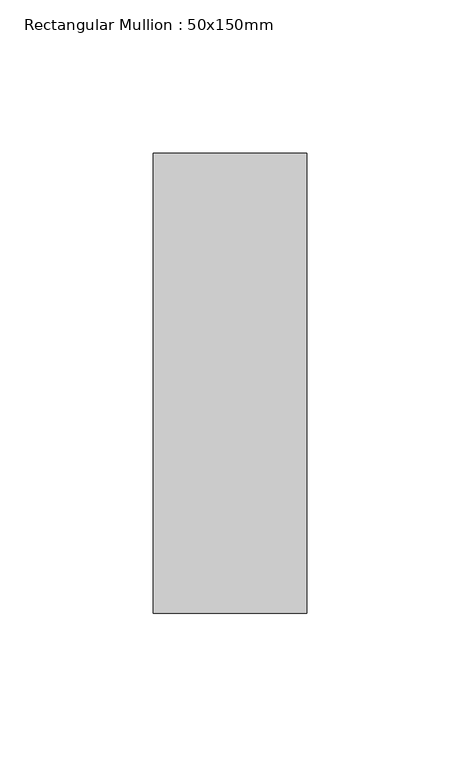
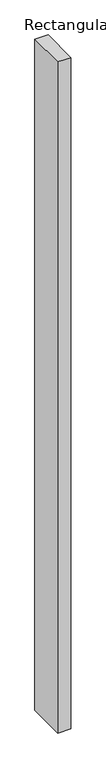
"""IFC4 building model written with IfcOpenShell, lengths in millimetres: member geometry, Rectangular Mullion : 50x150mm."""

import ifcopenshell
import ifcopenshell.guid

model = None  # the IFC model being written
_history = None  # IfcOwnerHistory: only IFC2X3 demands one
_inside = {}  # id of a spatial element -> (the spatial element, [elements in it])
_under = {}  # id of a project, library or spatial element -> (it, [spatial elements below it])
_declared = {}  # id of a project -> (the project, [libraries it declares])
_typed = {}  # id of a type object -> (the type object, [elements of that type])
_made_of = {}  # id of a material, layer set ... -> (it, [elements and type objects made of it])


def new_model(schema):
    """Start an empty IFC model of exactly this schema.

    Asked for "IFC4X3", IfcOpenShell would pick the latest addendum, in which some entities
    have other attributes; the version numbers below select the first issue.
    IFC2X3 requires an IfcOwnerHistory on every rooted entity: one is made here for all.
    """
    global model, _history
    if schema == "IFC4X3":
        model = ifcopenshell.file(schema_version=(4, 3, 0, 0))
    else:
        model = ifcopenshell.file(schema=schema)
    _inside.clear()
    _under.clear()
    _declared.clear()
    _typed.clear()
    _made_of.clear()
    _history = None
    if model.schema == "IFC2X3":
        org = make("IfcOrganization", Name="unknown")
        user = make(
            "IfcPersonAndOrganization",
            ThePerson=make("IfcPerson", FamilyName="unknown"),
            TheOrganization=org,
        )
        app = make(
            "IfcApplication",
            ApplicationDeveloper=org,
            Version="unknown",
            ApplicationFullName="unknown",
            ApplicationIdentifier="unknown",
        )
        _history = make(
            "IfcOwnerHistory",
            OwningUser=user,
            OwningApplication=app,
            ChangeAction="ADDED",
            CreationDate=0,
        )
    return model


def make(cls, **values):
    """One entity of the class cls with the attributes given. An attribute that is None is left unset."""
    return model.create_entity(
        cls, **{name: value for name, value in values.items() if value is not None}
    )


def rooted(cls, **values):
    """An entity with a GlobalId (a new one), such as an element, a storey or a relation."""
    return make(cls, GlobalId=ifcopenshell.guid.new(), OwnerHistory=_history, **values)


def si_unit(unit_type, name, prefix=None):
    """IfcSIUnit, for example si_unit("LENGTHUNIT", "METRE", prefix="MILLI")."""
    return make("IfcSIUnit", UnitType=unit_type, Prefix=prefix, Name=name)


def assignment(units):
    """IfcUnitAssignment: the units of a project."""
    return None if units is None else make("IfcUnitAssignment", Units=units)


def point(xyz):
    """IfcCartesianPoint."""
    return None if xyz is None else make("IfcCartesianPoint", Coordinates=xyz)


def direction(xyz):
    """IfcDirection."""
    return None if xyz is None else make("IfcDirection", DirectionRatios=xyz)


def frame(location, z_axis=None, x_axis=None):
    """IfcAxis2Placement3D, a coordinate frame: its origin and axes. An axis left out is left unset."""
    return make(
        "IfcAxis2Placement3D",
        Location=point(location),
        Axis=direction(z_axis),
        RefDirection=direction(x_axis),
    )


def origin():
    """The frame at (0, 0, 0) with its axes left unset."""
    return frame((0.0, 0.0, 0.0))


def place(relative_to, where):
    """IfcLocalPlacement: puts the frame where relative to a parent placement (None: the world)."""
    return make(
        "IfcLocalPlacement", PlacementRelTo=relative_to, RelativePlacement=where
    )


def context(
    kind, dimensions, precision=None, world=None, true_north=None, identifier=None
):
    """IfcGeometricRepresentationContext, for example the 3D "Model" context."""
    return make(
        "IfcGeometricRepresentationContext",
        ContextIdentifier=identifier,
        ContextType=kind,
        CoordinateSpaceDimension=dimensions,
        Precision=precision,
        WorldCoordinateSystem=world,
        TrueNorth=true_north,
    )


def project(units=None, contexts=None):
    """IfcProject with its units and contexts."""
    return rooted(
        "IfcProject",
        Name="project",
        RepresentationContexts=contexts,
        UnitsInContext=assignment(units),
    )


def spatial(cls, under=None, at=None, **own):
    """A site, building, storey or space (cls), placed at a placement, below another one or the project."""
    s = rooted(cls, ObjectPlacement=at, **own)
    if under is not None:
        _under.setdefault(under.id(), (under, []))[1].append(s)
    return s


def polyline(points):
    """IfcPolyline through the points."""
    return make("IfcPolyline", Points=[point(p) for p in points])


def outline(outer, holes=None, kind="AREA"):
    """IfcArbitraryClosedProfileDef: a profile drawn as a closed curve; with holes, ...WithVoids."""
    if holes is None:
        return make("IfcArbitraryClosedProfileDef", ProfileType=kind, OuterCurve=outer)
    return make(
        "IfcArbitraryProfileDefWithVoids",
        ProfileType=kind,
        OuterCurve=outer,
        InnerCurves=holes,
    )


def extrude(swept, where, along, depth):
    """IfcExtrudedAreaSolid: the profile swept, set in the frame where, extruded along a direction by depth."""
    return make(
        "IfcExtrudedAreaSolid",
        SweptArea=swept,
        Position=where,
        ExtrudedDirection=direction(along),
        Depth=depth,
    )


def shape(context_of_items, identifier, shape_type, items):
    """IfcShapeRepresentation: the items that make up one representation, for example the "Body"."""
    return make(
        "IfcShapeRepresentation",
        ContextOfItems=context_of_items,
        RepresentationIdentifier=identifier,
        RepresentationType=shape_type,
        Items=items,
    )


def source(mapping_origin, context_of_items, identifier, shape_type, items):
    """IfcRepresentationMap: a shape defined once, which mapped items show again and again."""
    return make(
        "IfcRepresentationMap",
        MappingOrigin=mapping_origin,
        MappedRepresentation=shape(context_of_items, identifier, shape_type, items),
    )


def transform(
    local_origin,
    x_axis=None,
    y_axis=None,
    z_axis=None,
    scale=None,
    scale2=None,
    scale3=None,
    uniform=True,
):
    """IfcCartesianTransformationOperator3D, or its non-uniform kind. x_axis, y_axis, z_axis: its Axis1, 2, 3."""
    if uniform:
        return make(
            "IfcCartesianTransformationOperator3D",
            Axis1=direction(x_axis),
            Axis2=direction(y_axis),
            LocalOrigin=point(local_origin),
            Scale=scale,
            Axis3=direction(z_axis),
        )
    return make(
        "IfcCartesianTransformationOperator3DnonUniform",
        Axis1=direction(x_axis),
        Axis2=direction(y_axis),
        LocalOrigin=point(local_origin),
        Scale=scale,
        Axis3=direction(z_axis),
        Scale2=scale2,
        Scale3=scale3,
    )


def mapped(mapping_source, mapping_target):
    """IfcMappedItem: shows the shape of a source again, moved by a transform."""
    return make(
        "IfcMappedItem", MappingSource=mapping_source, MappingTarget=mapping_target
    )


def made_of(thing, what):
    """Note that an element or type object is made of a material, layer set ...; save() writes the relation."""
    if what is not None:
        _made_of.setdefault(what.id(), (what, []))[1].append(thing)
    return thing


def element(
    cls,
    number,
    at=None,
    inside=None,
    cuts=None,
    type_object=None,
    material=None,
    context=None,
    identifier="Body",
    shape_type=None,
    held_by="IfcProductDefinitionShape",
    body=None,
    shapes=None,
    **own,
):
    """One element of the class cls, such as IfcWall. Its Tag is "e" and its number.

    at: its placement. inside: the storey or other place that contains it. cuts: it is an
    opening in that element (IfcRelVoidsElement). A single representation is given by context,
    identifier, shape_type and body (its items); several are given by shapes. held_by: the class
    of the entity that holds the representations. save() writes the other relations.
    """
    e = rooted(cls, Tag="e%d" % number, ObjectPlacement=at, **own)
    if body is not None:
        shapes = [shape(context, identifier, shape_type, body)]
    if shapes is not None:
        e.Representation = make(held_by, Representations=shapes)
    if inside is not None:
        _inside.setdefault(inside.id(), (inside, []))[1].append(e)
    if cuts is not None:
        rooted(
            "IfcRelVoidsElement", RelatingBuildingElement=cuts, RelatedOpeningElement=e
        )
    if type_object is not None:
        _typed.setdefault(type_object.id(), (type_object, []))[1].append(e)
    return made_of(e, material)


def aggregate(whole, parts):
    """IfcRelAggregates: a whole, such as a stair, and the parts it consists of."""
    return rooted("IfcRelAggregates", RelatingObject=whole, RelatedObjects=parts)


def save(model, path):
    """Write the relations noted so far, then the file.

    IfcRelAggregates (storeys below a building ...), IfcRelContainedInSpatialStructure (elements
    in a storey), IfcRelDefinesByType, IfcRelAssociatesMaterial and IfcRelDeclares: one each for
    every whole, place, type object, material and project.
    """
    for whole, parts in _under.values():
        aggregate(whole, parts)
    for where, things in _inside.values():
        rooted(
            "IfcRelContainedInSpatialStructure",
            RelatedElements=things,
            RelatingStructure=where,
        )
    for kind, things in _typed.values():
        rooted("IfcRelDefinesByType", RelatedObjects=things, RelatingType=kind)
    for what, things in _made_of.values():
        rooted("IfcRelAssociatesMaterial", RelatedObjects=things, RelatingMaterial=what)
    for by, libraries in _declared.values():
        rooted("IfcRelDeclares", RelatingContext=by, RelatedDefinitions=libraries)
    model.write(path)


def rectangular_mullion_50x150mm_929c4ac2(model_context):
    return source(origin(), model_context, "Body", "SweptSolid", [
        extrude(outline(polyline([(0.0, 75.0), (0.0, -75.0), (-50.0, -75.0), (-50.0, 75.0), (0.0, 75.0)])), frame((0.0, 0.0, -2700.0), z_axis=(0.0, 0.0, 1.0), x_axis=(1.0, 0.0, 0.0)), (0.0, 0.0, 1.0), 2700.0),
    ])


if __name__ == "__main__":
    model = new_model("IFC4")
    model_context = context("Model", 3, world=origin())
    ifc_project = project(units=[si_unit("LENGTHUNIT", "METRE", prefix="MILLI")], contexts=[model_context])
    site = spatial("IfcSite", under=ifc_project)
    building = spatial("IfcBuilding", under=site)
    placement = place(None, origin())
    rectangular_mullion_50x150mm_shape = rectangular_mullion_50x150mm_929c4ac2(model_context)
    element("IfcMember", 1, ObjectType="Rectangular Mullion : 50x150mm", at=placement, inside=building, context=model_context, shape_type="MappedRepresentation", body=[
        mapped(rectangular_mullion_50x150mm_shape, transform((0.0, 0.0, 0.0), x_axis=(1.0, 0.0, 0.0), y_axis=(0.0, 1.0, 0.0), z_axis=(0.0, 0.0, 1.0))),
    ])
    save(model, "model.ifc")

# Revit data of these elements
# Type "Rectangular Mullion : 50x150mm"
#   Keynote = "H11"
#   built-in parameter 1007304 = 0.492126 (stored number, unit not read)
#   built-in parameter 1007301 = 0.082021 (stored number, unit not read)
#   built-in parameter 1007300 = 0.082021 (stored number, unit not read)
# Element 1 (IfcMember, "Rectangular Mullion : 50x150mm")
#   Materials on its faces: "Aluminium"
# Materials
#   "Aluminium": class "Metal", colour RGB 247 247 247, transparency 0, Description = "Aluminium 6061", Cost = 0
